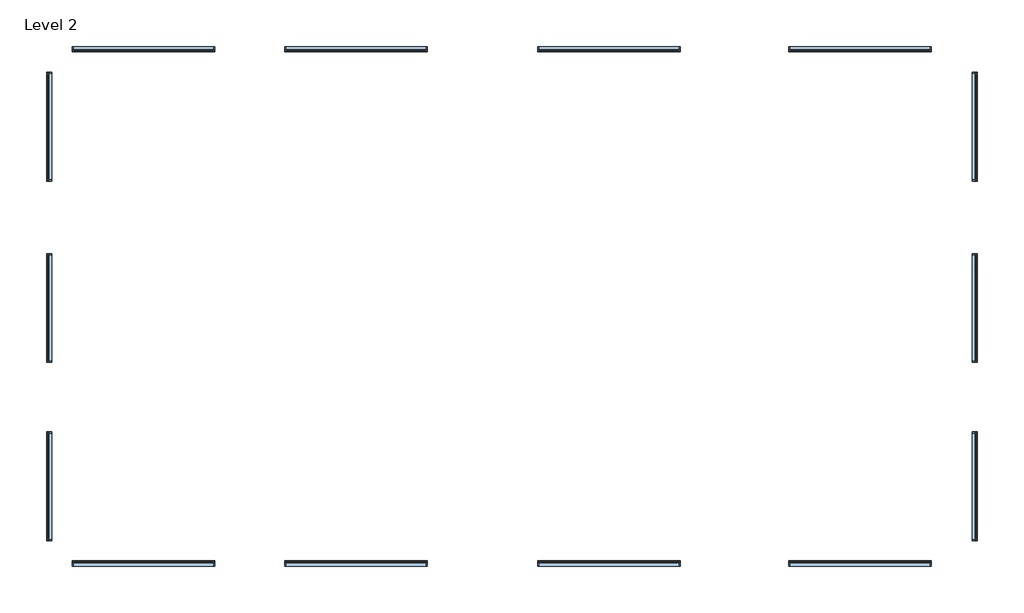
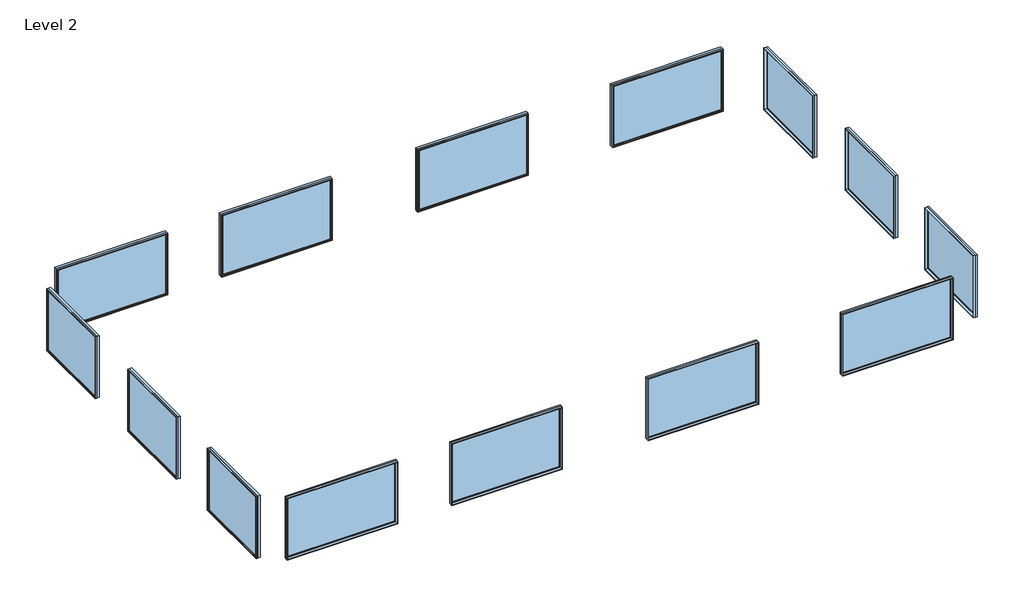
# One storey: 14 windows.
"""IFC4 building model written with IfcOpenShell, lengths in millimetres."""

import ifcopenshell
import ifcopenshell.guid

model = None  # the IFC model being written
_history = None  # IfcOwnerHistory: only IFC2X3 demands one
_inside = {}  # id of a spatial element -> (the spatial element, [elements in it])
_under = {}  # id of a project, library or spatial element -> (it, [spatial elements below it])
_declared = {}  # id of a project -> (the project, [libraries it declares])
_typed = {}  # id of a type object -> (the type object, [elements of that type])
_made_of = {}  # id of a material, layer set ... -> (it, [elements and type objects made of it])


def new_model(schema):
    """Start an empty IFC model of exactly this schema.

    Asked for "IFC4X3", IfcOpenShell would pick the latest addendum, in which some entities
    have other attributes; the version numbers below select the first issue.
    IFC2X3 requires an IfcOwnerHistory on every rooted entity: one is made here for all.
    """
    global model, _history
    if schema == "IFC4X3":
        model = ifcopenshell.file(schema_version=(4, 3, 0, 0))
    else:
        model = ifcopenshell.file(schema=schema)
    _inside.clear()
    _under.clear()
    _declared.clear()
    _typed.clear()
    _made_of.clear()
    _history = None
    if model.schema == "IFC2X3":
        org = make("IfcOrganization", Name="unknown")
        user = make(
            "IfcPersonAndOrganization",
            ThePerson=make("IfcPerson", FamilyName="unknown"),
            TheOrganization=org,
        )
        app = make(
            "IfcApplication",
            ApplicationDeveloper=org,
            Version="unknown",
            ApplicationFullName="unknown",
            ApplicationIdentifier="unknown",
        )
        _history = make(
            "IfcOwnerHistory",
            OwningUser=user,
            OwningApplication=app,
            ChangeAction="ADDED",
            CreationDate=0,
        )
    return model


def make(cls, **values):
    """One entity of the class cls with the attributes given. An attribute that is None is left unset."""
    return model.create_entity(
        cls, **{name: value for name, value in values.items() if value is not None}
    )


def rooted(cls, **values):
    """An entity with a GlobalId (a new one), such as an element, a storey or a relation."""
    return make(cls, GlobalId=ifcopenshell.guid.new(), OwnerHistory=_history, **values)


def si_unit(unit_type, name, prefix=None):
    """IfcSIUnit, for example si_unit("LENGTHUNIT", "METRE", prefix="MILLI")."""
    return make("IfcSIUnit", UnitType=unit_type, Prefix=prefix, Name=name)


def assignment(units):
    """IfcUnitAssignment: the units of a project."""
    return None if units is None else make("IfcUnitAssignment", Units=units)


def point(xyz):
    """IfcCartesianPoint."""
    return None if xyz is None else make("IfcCartesianPoint", Coordinates=xyz)


def direction(xyz):
    """IfcDirection."""
    return None if xyz is None else make("IfcDirection", DirectionRatios=xyz)


def frame(location, z_axis=None, x_axis=None):
    """IfcAxis2Placement3D, a coordinate frame: its origin and axes. An axis left out is left unset."""
    return make(
        "IfcAxis2Placement3D",
        Location=point(location),
        Axis=direction(z_axis),
        RefDirection=direction(x_axis),
    )


def origin():
    """The frame at (0, 0, 0) with its axes left unset."""
    return frame((0.0, 0.0, 0.0))


def place(relative_to, where):
    """IfcLocalPlacement: puts the frame where relative to a parent placement (None: the world)."""
    return make(
        "IfcLocalPlacement", PlacementRelTo=relative_to, RelativePlacement=where
    )


def context(
    kind, dimensions, precision=None, world=None, true_north=None, identifier=None
):
    """IfcGeometricRepresentationContext, for example the 3D "Model" context."""
    return make(
        "IfcGeometricRepresentationContext",
        ContextIdentifier=identifier,
        ContextType=kind,
        CoordinateSpaceDimension=dimensions,
        Precision=precision,
        WorldCoordinateSystem=world,
        TrueNorth=true_north,
    )


def project(units=None, contexts=None):
    """IfcProject with its units and contexts."""
    return rooted(
        "IfcProject",
        Name="project",
        RepresentationContexts=contexts,
        UnitsInContext=assignment(units),
    )


def spatial(cls, under=None, at=None, **own):
    """A site, building, storey or space (cls), placed at a placement, below another one or the project."""
    s = rooted(cls, ObjectPlacement=at, **own)
    if under is not None:
        _under.setdefault(under.id(), (under, []))[1].append(s)
    return s


def polyline(points):
    """IfcPolyline through the points."""
    return make("IfcPolyline", Points=[point(p) for p in points])


def outline(outer, holes=None, kind="AREA"):
    """IfcArbitraryClosedProfileDef: a profile drawn as a closed curve; with holes, ...WithVoids."""
    if holes is None:
        return make("IfcArbitraryClosedProfileDef", ProfileType=kind, OuterCurve=outer)
    return make(
        "IfcArbitraryProfileDefWithVoids",
        ProfileType=kind,
        OuterCurve=outer,
        InnerCurves=holes,
    )


def extrude(swept, where, along, depth):
    """IfcExtrudedAreaSolid: the profile swept, set in the frame where, extruded along a direction by depth."""
    return make(
        "IfcExtrudedAreaSolid",
        SweptArea=swept,
        Position=where,
        ExtrudedDirection=direction(along),
        Depth=depth,
    )


def shape(context_of_items, identifier, shape_type, items):
    """IfcShapeRepresentation: the items that make up one representation, for example the "Body"."""
    return make(
        "IfcShapeRepresentation",
        ContextOfItems=context_of_items,
        RepresentationIdentifier=identifier,
        RepresentationType=shape_type,
        Items=items,
    )


def source(mapping_origin, context_of_items, identifier, shape_type, items):
    """IfcRepresentationMap: a shape defined once, which mapped items show again and again."""
    return make(
        "IfcRepresentationMap",
        MappingOrigin=mapping_origin,
        MappedRepresentation=shape(context_of_items, identifier, shape_type, items),
    )


def transform(
    local_origin,
    x_axis=None,
    y_axis=None,
    z_axis=None,
    scale=None,
    scale2=None,
    scale3=None,
    uniform=True,
):
    """IfcCartesianTransformationOperator3D, or its non-uniform kind. x_axis, y_axis, z_axis: its Axis1, 2, 3."""
    if uniform:
        return make(
            "IfcCartesianTransformationOperator3D",
            Axis1=direction(x_axis),
            Axis2=direction(y_axis),
            LocalOrigin=point(local_origin),
            Scale=scale,
            Axis3=direction(z_axis),
        )
    return make(
        "IfcCartesianTransformationOperator3DnonUniform",
        Axis1=direction(x_axis),
        Axis2=direction(y_axis),
        LocalOrigin=point(local_origin),
        Scale=scale,
        Axis3=direction(z_axis),
        Scale2=scale2,
        Scale3=scale3,
    )


def mapped(mapping_source, mapping_target):
    """IfcMappedItem: shows the shape of a source again, moved by a transform."""
    return make(
        "IfcMappedItem", MappingSource=mapping_source, MappingTarget=mapping_target
    )


def made_of(thing, what):
    """Note that an element or type object is made of a material, layer set ...; save() writes the relation."""
    if what is not None:
        _made_of.setdefault(what.id(), (what, []))[1].append(thing)
    return thing


def element(
    cls,
    number,
    at=None,
    inside=None,
    cuts=None,
    type_object=None,
    material=None,
    context=None,
    identifier="Body",
    shape_type=None,
    held_by="IfcProductDefinitionShape",
    body=None,
    shapes=None,
    **own,
):
    """One element of the class cls, such as IfcWall. Its Tag is "e" and its number.

    at: its placement. inside: the storey or other place that contains it. cuts: it is an
    opening in that element (IfcRelVoidsElement). A single representation is given by context,
    identifier, shape_type and body (its items); several are given by shapes. held_by: the class
    of the entity that holds the representations. save() writes the other relations.
    """
    e = rooted(cls, Tag="e%d" % number, ObjectPlacement=at, **own)
    if body is not None:
        shapes = [shape(context, identifier, shape_type, body)]
    if shapes is not None:
        e.Representation = make(held_by, Representations=shapes)
    if inside is not None:
        _inside.setdefault(inside.id(), (inside, []))[1].append(e)
    if cuts is not None:
        rooted(
            "IfcRelVoidsElement", RelatingBuildingElement=cuts, RelatedOpeningElement=e
        )
    if type_object is not None:
        _typed.setdefault(type_object.id(), (type_object, []))[1].append(e)
    return made_of(e, material)


def aggregate(whole, parts):
    """IfcRelAggregates: a whole, such as a stair, and the parts it consists of."""
    return rooted("IfcRelAggregates", RelatingObject=whole, RelatedObjects=parts)


def save(model, path):
    """Write the relations noted so far, then the file.

    IfcRelAggregates (storeys below a building ...), IfcRelContainedInSpatialStructure (elements
    in a storey), IfcRelDefinesByType, IfcRelAssociatesMaterial and IfcRelDeclares: one each for
    every whole, place, type object, material and project.
    """
    for whole, parts in _under.values():
        aggregate(whole, parts)
    for where, things in _inside.values():
        rooted(
            "IfcRelContainedInSpatialStructure",
            RelatedElements=things,
            RelatingStructure=where,
        )
    for kind, things in _typed.values():
        rooted("IfcRelDefinesByType", RelatedObjects=things, RelatingType=kind)
    for what, things in _made_of.values():
        rooted("IfcRelAssociatesMaterial", RelatedObjects=things, RelatingMaterial=what)
    for by, libraries in _declared.values():
        rooted("IfcRelDeclares", RelatingContext=by, RelatedDefinitions=libraries)
    model.write(path)


def m_fixed_2500x_4228mm_fd5e51e7(model_context):
    return source(origin(), model_context, "Body", "SweptSolid", [
        extrude(outline(polyline([(-2050.8, 54.2), (2050.8, 54.2), (2050.8, 42.2), (-2050.8, 42.2), (-2050.8, 54.2)])), frame((0.0, 0.0, 368.0), z_axis=(0.0, 0.0, 1.0), x_axis=(1.0, 0.0, 0.0)), (0.0, 0.0, 1.0), 2374.0),
        extrude(outline(polyline([(2786.0, -2094.8), (324.0, -2094.8), (324.0, 2094.8), (2786.0, 2094.8), (2786.0, -2094.8)]), holes=[polyline([(2742.0, -2050.8), (2742.0, 2050.8), (368.0, 2050.8), (368.0, -2050.8), (2742.0, -2050.8)])]), frame((0.0, 26.2, 0.0), z_axis=(0.0, 1.0, 0.0), x_axis=(0.0, 0.0, 1.0)), (0.0, 0.0, 1.0), 44.0),
        extrude(outline(polyline([(2805.0, -2113.8), (305.0, -2113.8), (305.0, 2113.8), (2805.0, 2113.8), (2805.0, -2113.8)]), holes=[polyline([(2786.0, -2094.8), (2786.0, 2094.8), (324.0, 2094.8), (324.0, -2094.8), (2786.0, -2094.8)])]), frame((0.0, 26.2, 0.0), z_axis=(0.0, 1.0, 0.0), x_axis=(0.0, 0.0, 1.0)), (0.0, 0.0, 1.0), 63.0),
        extrude(outline(polyline([(2805.0, -2113.8), (305.0, -2113.8), (305.0, 2113.8), (2805.0, 2113.8), (2805.0, -2113.8)]), holes=[polyline([(2773.0, -2081.8), (2773.0, 2081.8), (337.0, 2081.8), (337.0, -2081.8), (2773.0, -2081.8)])]), frame((0.0, -63.2, 0.0), z_axis=(0.0, 1.0, 0.0), x_axis=(0.0, 0.0, 1.0)), (0.0, 0.0, 1.0), 89.4),
    ])


def m_fixed_2500x_4228mm_f14c179f(model_context):
    return source(origin(), model_context, "Body", "SweptSolid", [
        extrude(outline(polyline([(-2050.8, -54.2), (-2050.8, -42.2), (2050.8, -42.2), (2050.8, -54.2), (-2050.8, -54.2)])), frame((0.0, 0.0, 368.0), z_axis=(0.0, 0.0, 1.0), x_axis=(1.0, 0.0, 0.0)), (0.0, 0.0, 1.0), 2374.0),
        extrude(outline(polyline([(2786.0, -2094.8), (324.0, -2094.8), (324.0, 2094.8), (2786.0, 2094.8), (2786.0, -2094.8)]), holes=[polyline([(2742.0, -2050.8), (2742.0, 2050.8), (368.0, 2050.8), (368.0, -2050.8), (2742.0, -2050.8)])]), frame((0.0, -70.2, 0.0), z_axis=(0.0, 1.0, 0.0), x_axis=(0.0, 0.0, 1.0)), (0.0, 0.0, 1.0), 44.0),
        extrude(outline(polyline([(2805.0, -2113.8), (305.0, -2113.8), (305.0, 2113.8), (2805.0, 2113.8), (2805.0, -2113.8)]), holes=[polyline([(2786.0, -2094.8), (2786.0, 2094.8), (324.0, 2094.8), (324.0, -2094.8), (2786.0, -2094.8)])]), frame((0.0, -89.2, 0.0), z_axis=(0.0, 1.0, 0.0), x_axis=(0.0, 0.0, 1.0)), (0.0, 0.0, 1.0), 63.0),
        extrude(outline(polyline([(2805.0, -2113.8), (305.0, -2113.8), (305.0, 2113.8), (2805.0, 2113.8), (2805.0, -2113.8)]), holes=[polyline([(2773.0, -2081.8), (2773.0, 2081.8), (337.0, 2081.8), (337.0, -2081.8), (2773.0, -2081.8)])]), frame((0.0, -26.2, 0.0), z_axis=(0.0, 1.0, 0.0), x_axis=(0.0, 0.0, 1.0)), (0.0, 0.0, 1.0), 89.4),
    ])


def m_fixed_2500x_3220mm_df94f4d0(model_context):
    return source(origin(), model_context, "Body", "SweptSolid", [
        extrude(outline(polyline([(-1546.8, 54.2), (1546.8, 54.2), (1546.8, 42.2), (-1546.8, 42.2), (-1546.8, 54.2)])), frame((0.0, 0.0, 368.0), z_axis=(0.0, 0.0, 1.0), x_axis=(1.0, 0.0, 0.0)), (0.0, 0.0, 1.0), 2374.0),
        extrude(outline(polyline([(2786.0, -1590.8), (324.0, -1590.8), (324.0, 1590.8), (2786.0, 1590.8), (2786.0, -1590.8)]), holes=[polyline([(2742.0, -1546.8), (2742.0, 1546.8), (368.0, 1546.8), (368.0, -1546.8), (2742.0, -1546.8)])]), frame((0.0, 26.2, 0.0), z_axis=(0.0, 1.0, 0.0), x_axis=(0.0, 0.0, 1.0)), (0.0, 0.0, 1.0), 44.0),
        extrude(outline(polyline([(2805.0, -1609.8), (305.0, -1609.8), (305.0, 1609.8), (2805.0, 1609.8), (2805.0, -1609.8)]), holes=[polyline([(2786.0, -1590.8), (2786.0, 1590.8), (324.0, 1590.8), (324.0, -1590.8), (2786.0, -1590.8)])]), frame((0.0, 26.2, 0.0), z_axis=(0.0, 1.0, 0.0), x_axis=(0.0, 0.0, 1.0)), (0.0, 0.0, 1.0), 63.0),
        extrude(outline(polyline([(2805.0, -1609.8), (305.0, -1609.8), (305.0, 1609.8), (2805.0, 1609.8), (2805.0, -1609.8)]), holes=[polyline([(2773.0, -1577.8), (2773.0, 1577.8), (337.0, 1577.8), (337.0, -1577.8), (2773.0, -1577.8)])]), frame((0.0, -63.2, 0.0), z_axis=(0.0, 1.0, 0.0), x_axis=(0.0, 0.0, 1.0)), (0.0, 0.0, 1.0), 89.4),
    ])


def m_fixed_2500x_3220mm_8b997f8c(model_context):
    return source(origin(), model_context, "Body", "SweptSolid", [
        extrude(outline(polyline([(-1546.8, -54.2), (-1546.8, -42.2), (1546.8, -42.2), (1546.8, -54.2), (-1546.8, -54.2)])), frame((0.0, 0.0, 368.0), z_axis=(0.0, 0.0, 1.0), x_axis=(1.0, 0.0, 0.0)), (0.0, 0.0, 1.0), 2374.0),
        extrude(outline(polyline([(2786.0, -1590.8), (324.0, -1590.8), (324.0, 1590.8), (2786.0, 1590.8), (2786.0, -1590.8)]), holes=[polyline([(2742.0, -1546.8), (2742.0, 1546.8), (368.0, 1546.8), (368.0, -1546.8), (2742.0, -1546.8)])]), frame((0.0, -70.2, 0.0), z_axis=(0.0, 1.0, 0.0), x_axis=(0.0, 0.0, 1.0)), (0.0, 0.0, 1.0), 44.0),
        extrude(outline(polyline([(2805.0, -1609.8), (305.0, -1609.8), (305.0, 1609.8), (2805.0, 1609.8), (2805.0, -1609.8)]), holes=[polyline([(2786.0, -1590.8), (2786.0, 1590.8), (324.0, 1590.8), (324.0, -1590.8), (2786.0, -1590.8)])]), frame((0.0, -89.2, 0.0), z_axis=(0.0, 1.0, 0.0), x_axis=(0.0, 0.0, 1.0)), (0.0, 0.0, 1.0), 63.0),
        extrude(outline(polyline([(2805.0, -1609.8), (305.0, -1609.8), (305.0, 1609.8), (2805.0, 1609.8), (2805.0, -1609.8)]), holes=[polyline([(2773.0, -1577.8), (2773.0, 1577.8), (337.0, 1577.8), (337.0, -1577.8), (2773.0, -1577.8)])]), frame((0.0, -26.2, 0.0), z_axis=(0.0, 1.0, 0.0), x_axis=(0.0, 0.0, 1.0)), (0.0, 0.0, 1.0), 89.4),
    ])


model = new_model("IFC4")

# Units and contexts
model_context = context("Model", 3, world=origin())
ifc_project = project(units=[si_unit("LENGTHUNIT", "METRE", prefix="MILLI")], contexts=[model_context])

# Site, building, storey
site = spatial("IfcSite", under=ifc_project)
building = spatial("IfcBuilding", under=site)
storey = spatial("IfcBuildingStorey", under=building, Name="Level 2", Elevation=3962.4)

# Windows
placement = place(None, origin())
m_fixed_2500x_4228mm_shape = m_fixed_2500x_4228mm_fd5e51e7(model_context)
element("IfcWindow", 1, ObjectType="M_Fixed : 2500X 4228mm", at=placement, inside=storey, context=model_context, shape_type="MappedRepresentation", body=[
    mapped(m_fixed_2500x_4228mm_shape, transform((4360.264681, 11233.7802217, 4557.4), x_axis=(-1.0, 0.0, 0.0), y_axis=(0.0, -1.0, 0.0), z_axis=(0.0, 0.0, 1.0))),
])
element("IfcWindow", 2, ObjectType="M_Fixed : 2500X 4228mm", at=placement, inside=storey, context=model_context, shape_type="MappedRepresentation", body=[
    mapped(m_fixed_2500x_4228mm_shape, transform((10652.264681, 11233.7802217, 4557.4), x_axis=(-1.0, 0.0, 0.0), y_axis=(0.0, -1.0, 0.0), z_axis=(0.0, 0.0, 1.0))),
])
element("IfcWindow", 3, ObjectType="M_Fixed : 2500X 4228mm", at=placement, inside=storey, context=model_context, shape_type="MappedRepresentation", body=[
    mapped(m_fixed_2500x_4228mm_shape, transform((18152.264681, 11233.7802217, 4557.4), x_axis=(-1.0, 0.0, 0.0), y_axis=(0.0, -1.0, 0.0), z_axis=(0.0, 0.0, 1.0))),
])
element("IfcWindow", 4, ObjectType="M_Fixed : 2500X 4228mm", at=placement, inside=storey, context=model_context, shape_type="MappedRepresentation", body=[
    mapped(m_fixed_2500x_4228mm_shape, transform((25592.264681, 11233.7802217, 4557.4), x_axis=(-1.0, 0.0, 0.0), y_axis=(0.0, -1.0, 0.0), z_axis=(0.0, 0.0, 1.0))),
])
m_fixed_2500x_4228mm_2_shape = m_fixed_2500x_4228mm_f14c179f(model_context)
element("IfcWindow", 5, ObjectType="M_Fixed : 2500X 4228mm", at=placement, inside=storey, context=model_context, shape_type="MappedRepresentation", body=[
    mapped(m_fixed_2500x_4228mm_2_shape, transform((4360.264681, -4032.2197783, 4557.4), x_axis=(-1.0, 0.0, 0.0), y_axis=(0.0, -1.0, 0.0), z_axis=(0.0, 0.0, 1.0))),
])
element("IfcWindow", 6, ObjectType="M_Fixed : 2500X 4228mm", at=placement, inside=storey, context=model_context, shape_type="MappedRepresentation", body=[
    mapped(m_fixed_2500x_4228mm_2_shape, transform((10652.264681, -4032.2197783, 4557.4), x_axis=(-1.0, 0.0, 0.0), y_axis=(0.0, -1.0, 0.0), z_axis=(0.0, 0.0, 1.0))),
])
element("IfcWindow", 7, ObjectType="M_Fixed : 2500X 4228mm", at=placement, inside=storey, context=model_context, shape_type="MappedRepresentation", body=[
    mapped(m_fixed_2500x_4228mm_2_shape, transform((18152.264681, -4032.2197783, 4557.4), x_axis=(-1.0, 0.0, 0.0), y_axis=(0.0, -1.0, 0.0), z_axis=(0.0, 0.0, 1.0))),
])
element("IfcWindow", 8, ObjectType="M_Fixed : 2500X 4228mm", at=placement, inside=storey, context=model_context, shape_type="MappedRepresentation", body=[
    mapped(m_fixed_2500x_4228mm_2_shape, transform((25592.264681, -4032.2197783, 4557.4), x_axis=(-1.0, 0.0, 0.0), y_axis=(0.0, -1.0, 0.0), z_axis=(0.0, 0.0, 1.0))),
])
m_fixed_2500x_3220mm_shape = m_fixed_2500x_3220mm_df94f4d0(model_context)
element("IfcWindow", 9, ObjectType="M_Fixed : 2500x 3220mm", at=placement, inside=storey, context=model_context, shape_type="MappedRepresentation", body=[
    mapped(m_fixed_2500x_3220mm_shape, transform((1573.264681, 8920.7802217, 4429.5029682), x_axis=(0.0, 1.0, 0.0), y_axis=(-1.0, 0.0, 0.0), z_axis=(0.0, 0.0, 1.0))),
])
element("IfcWindow", 10, ObjectType="M_Fixed : 2500x 3220mm", at=placement, inside=storey, context=model_context, shape_type="MappedRepresentation", body=[
    mapped(m_fixed_2500x_3220mm_shape, transform((1573.264681, 3552.7802217, 4429.5029682), x_axis=(0.0, 1.0, 0.0), y_axis=(-1.0, 0.0, 0.0), z_axis=(0.0, 0.0, 1.0))),
])
element("IfcWindow", 11, ObjectType="M_Fixed : 2500x 3220mm", at=placement, inside=storey, context=model_context, shape_type="MappedRepresentation", body=[
    mapped(m_fixed_2500x_3220mm_shape, transform((1573.264681, -1733.2197783, 4429.5029682), x_axis=(0.0, 1.0, 0.0), y_axis=(-1.0, 0.0, 0.0), z_axis=(0.0, 0.0, 1.0))),
])
m_fixed_2500x_3220mm_2_shape = m_fixed_2500x_3220mm_8b997f8c(model_context)
element("IfcWindow", 12, ObjectType="M_Fixed : 2500x 3220mm", at=placement, inside=storey, context=model_context, shape_type="MappedRepresentation", body=[
    mapped(m_fixed_2500x_3220mm_2_shape, transform((28979.264681, 8920.7802217, 4559.8), x_axis=(0.0, 1.0, 0.0), y_axis=(-1.0, 0.0, 0.0), z_axis=(0.0, 0.0, 1.0))),
])
element("IfcWindow", 13, ObjectType="M_Fixed : 2500x 3220mm", at=placement, inside=storey, context=model_context, shape_type="MappedRepresentation", body=[
    mapped(m_fixed_2500x_3220mm_2_shape, transform((28979.264681, 3552.7802217, 4559.8), x_axis=(0.0, 1.0, 0.0), y_axis=(-1.0, 0.0, 0.0), z_axis=(0.0, 0.0, 1.0))),
])
element("IfcWindow", 14, ObjectType="M_Fixed : 2500x 3220mm", at=placement, inside=storey, context=model_context, shape_type="MappedRepresentation", body=[
    mapped(m_fixed_2500x_3220mm_2_shape, transform((28979.264681, -1733.2197783, 4559.8), x_axis=(0.0, 1.0, 0.0), y_axis=(-1.0, 0.0, 0.0), z_axis=(0.0, 0.0, 1.0))),
])

save(model, "model.ifc")

# Revit data of these elements
# Type "M_Fixed : 2500X 4228mm"
#   Type Mark = "25"
#   Height = 2500 mm
#   Default Sill Height = 305 mm
#   Width = 4227.6 mm
#   Window Inset = 19 mm
#   Frame Exterior Material = Sash
#   Frame Interior Material = Sash
#   Glass Pane Material = Glass
#   Sash = Sash
#   Wall Closure = (empty or 0)
# Type "M_Fixed : 2500x 3220mm"
#   Type Mark = "26"
#   Height = 2500 mm
#   Default Sill Height = 305 mm
#   Width = 3219.6 mm
#   Window Inset = 19 mm
#   Frame Exterior Material = Sash
#   Frame Interior Material = Sash
#   Glass Pane Material = Glass
#   Sash = Sash
#   Wall Closure = (empty or 0)
# Element 1 (IfcWindow, "M_Fixed : 2500X 4228mm")
#   Mark = "1"
#   Phase Created = New Construction
#   Materials on its faces: "Sash", "Glass"
# Element 2 (IfcWindow, "M_Fixed : 2500X 4228mm")
#   Mark = "2"
#   Phase Created = New Construction
#   Materials on its faces: "Sash", "Glass"
# Element 3 (IfcWindow, "M_Fixed : 2500X 4228mm")
#   Mark = "3"
#   Phase Created = New Construction
#   Materials on its faces: "Sash", "Glass"
# Element 4 (IfcWindow, "M_Fixed : 2500X 4228mm")
#   Mark = "4"
#   Phase Created = New Construction
#   Materials on its faces: "Sash", "Glass"
# Element 5 (IfcWindow, "M_Fixed : 2500X 4228mm")
#   Mark = "5"
#   Phase Created = New Construction
#   Materials on its faces: "Sash", "Glass"
# Element 6 (IfcWindow, "M_Fixed : 2500X 4228mm")
#   Mark = "6"
#   Phase Created = New Construction
#   Materials on its faces: "Sash", "Glass"
# Element 7 (IfcWindow, "M_Fixed : 2500X 4228mm")
#   Mark = "7"
#   Phase Created = New Construction
#   Materials on its faces: "Sash", "Glass"
# Element 8 (IfcWindow, "M_Fixed : 2500X 4228mm")
#   Mark = "8"
#   Phase Created = New Construction
#   Materials on its faces: "Sash", "Glass"
# Element 9 (IfcWindow, "M_Fixed : 2500x 3220mm")
#   Mark = "23"
#   Phase Created = New Construction
#   Materials on its faces: "Sash", "Glass"
# Element 10 (IfcWindow, "M_Fixed : 2500x 3220mm")
#   Mark = "24"
#   Phase Created = New Construction
#   Materials on its faces: "Sash", "Glass"
# Element 11 (IfcWindow, "M_Fixed : 2500x 3220mm")
#   Mark = "25"
#   Phase Created = New Construction
#   Materials on its faces: "Sash", "Glass"
# Element 12 (IfcWindow, "M_Fixed : 2500x 3220mm")
#   Mark = "20"
#   Phase Created = New Construction
#   Materials on its faces: "Sash", "Glass"
# Element 13 (IfcWindow, "M_Fixed : 2500x 3220mm")
#   Mark = "21"
#   Phase Created = New Construction
#   Materials on its faces: "Sash", "Glass"
# Element 14 (IfcWindow, "M_Fixed : 2500x 3220mm")
#   Mark = "22"
#   Phase Created = New Construction
#   Materials on its faces: "Sash", "Glass"
# Materials
#   "Sash": class "Wood", colour RGB 136 99 55, transparency 0
#   "Glass": class "Glass", colour RGB 0 128 192, transparency 0.9, Description = "Soda Lime Glass", Cost = 0
# Room at (7702.307, 8283.876) mm, phase "New Construction", upper level "Roof Level", upper offset 0 mm, lower offset 0 mm
#   Number = "9"
#   Name = "Room"
# Room at (8641.307, 981.272) mm, phase "New Construction", upper level "Roof Level", upper offset 0 mm, lower offset 0 mm
#   Number = "10"
#   Name = "Room"
